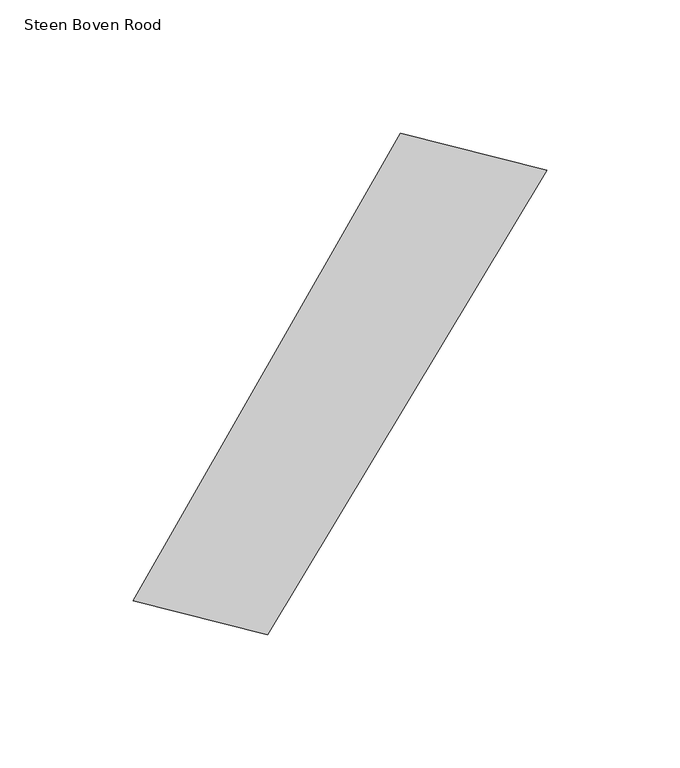
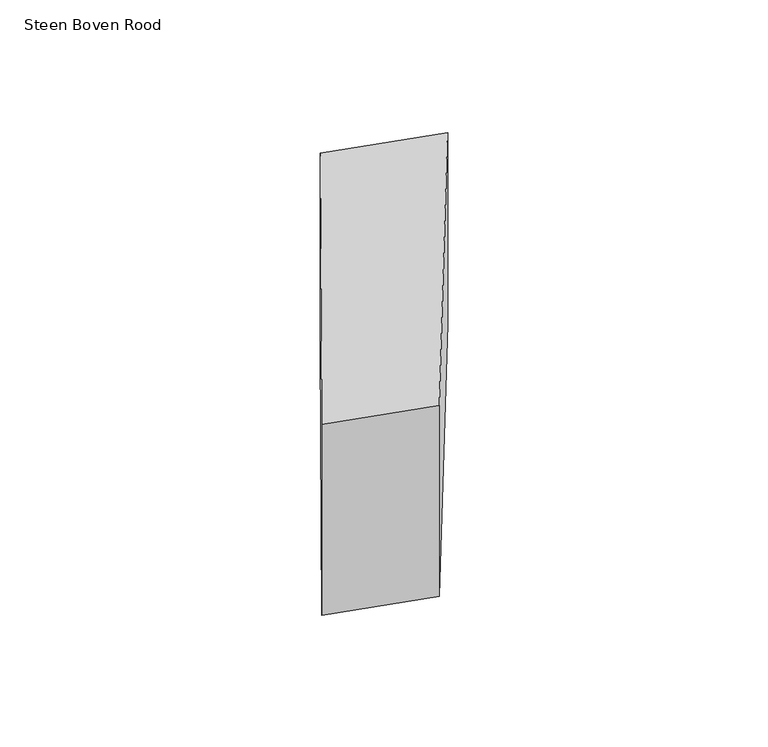
"""IFC4 building model written with IfcOpenShell, lengths in millimetres: proxy geometry, 00_GMA_steen_versie_4 : Steen Boven Rood."""

from ifc_helpers import new_model, si_unit, origin, origin_with_axes, place, context, project, spatial, polyline, outline, extrude, source, transform, mapped, element, save


def steen_boven_rood_4cad9197(model_context):
    return source(origin(), model_context, "Body", "SweptSolid", [
        extrude(outline(polyline([(154.4756475, 159.3243939), (49.5159473, -15.373942), (-1.1781711, -2.4291705), (99.5643276, 173.3193236), (154.4756475, 159.3243939)])), origin_with_axes(), (0.0, 0.0, 1.0), 100.0),
    ])


if __name__ == "__main__":
    model = new_model("IFC4")
    model_context = context("Model", 3, world=origin())
    ifc_project = project(units=[si_unit("LENGTHUNIT", "METRE", prefix="MILLI")], contexts=[model_context])
    site = spatial("IfcSite", under=ifc_project)
    building = spatial("IfcBuilding", under=site)
    placement = place(None, origin())
    steen_boven_rood_shape = steen_boven_rood_4cad9197(model_context)
    element("IfcBuildingElementProxy", 1, Name="00_GMA_steen_versie_4 : Steen Boven Rood", ObjectType="00_GMA_steen_versie_4 : Steen Boven Rood", at=placement, inside=building, context=model_context, shape_type="MappedRepresentation", body=[
        mapped(steen_boven_rood_shape, transform((0.0, 0.0, 0.0), x_axis=(1.0, 0.0, 0.0), y_axis=(0.0, 1.0, 0.0), z_axis=(0.0, 0.0, 1.0))),
    ])
    save(model, "model.ifc")

# Revit data of these elements
# Type "00_GMA_steen_versie_4 : Steen Boven Rood"
#   StootVoegHalfBoven [instance default] = 5 mm
#   StootVoegHalf [instance default] = 5 mm
#   StootVoegBreedteOnder = 10 mm
#   StootVoegBreedteBoven = 10 mm
#   Steendikte = 100 mm
#   LintVoegOnderHalf = 5 mm
#   LintVoegOnder = 10 mm
#   LintVoegBovenHalf = 0 mm
#   LintVoegBoven = 0 mm
#   materiaal = 21_steen_rood
#   MateriaalVoeg = none
#   Default Elevation = 0
# Element 1 (IfcBuildingElementProxy, "00_GMA_steen_versie_4 : Steen Boven Rood")
#   Materials on its faces: "21_steen_rood"
# Materials
#   "21_steen_rood": class "Unassigned", colour RGB 213 111 43, transparency 0, Cost = 0
